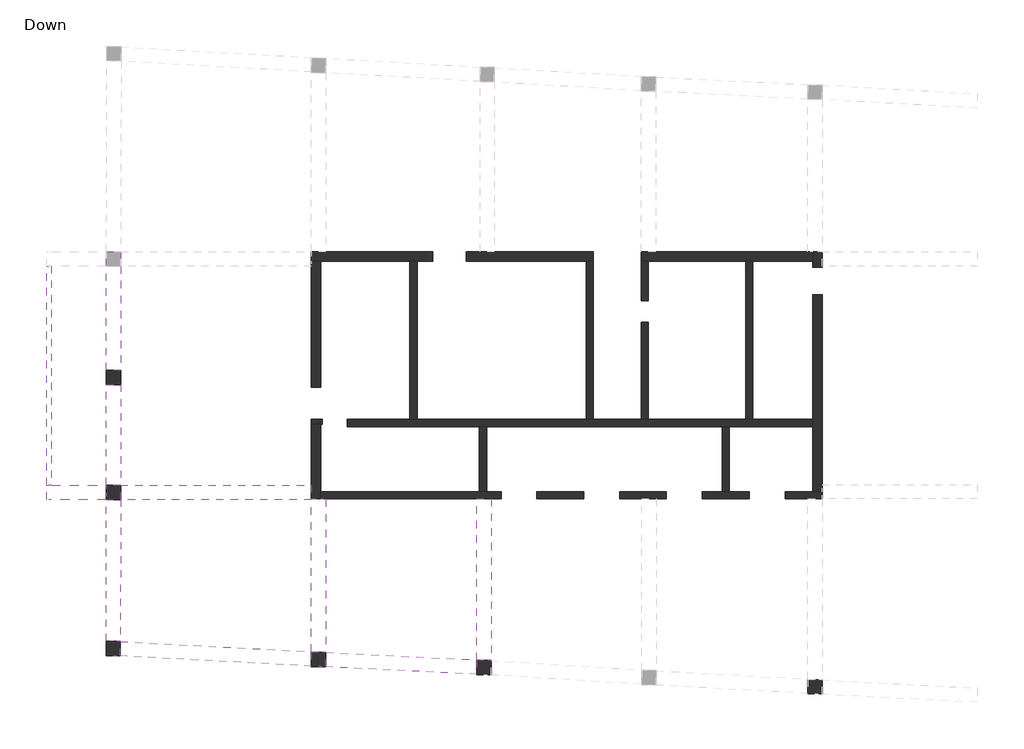
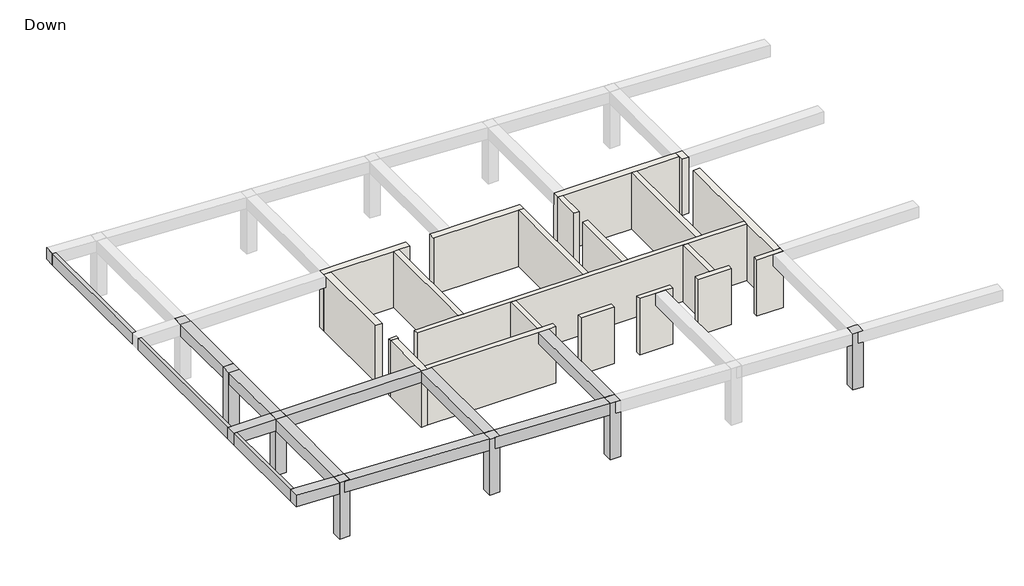
# One storey, part 1 of 2: 21 walls, 10 beams, 6 columns.
"""IFC4 building model written with IfcOpenShell, lengths in millimetres."""

from ifc_helpers import new_model, si_unit, origin, origin_with_axes, place, context, project, spatial, polyline, outline, extrude, faceted_brep, element, save

model = new_model("IFC4")

# Units and contexts
model_context = context("Model", 3, world=origin())
ifc_project = project(units=[si_unit("LENGTHUNIT", "METRE", prefix="MILLI")], contexts=[model_context])

# Site, building, storey
site = spatial("IfcSite", under=ifc_project)
building = spatial("IfcBuilding", under=site)
storey = spatial("IfcBuildingStorey", under=building, Name="Down", Elevation=0.0)

# Beams
placement = place(None, origin())
element("IfcBeam", 1, ObjectType="Concrete Rectengular Beam : 20/70", at=placement, inside=storey, context=model_context, shape_type="Brep", body=[
    faceted_brep([(-18610.0734048, 10852.5835779, 3500.0), (-18643.7818749, 10854.4803419, 3500.0), (-18643.7818749, 10253.5312104, 3500.0), (-18443.7818749, 10242.2772794, 2800.0), (-18443.7818749, 10242.2772794, 3250.0), (-18443.7818749, 10242.2772794, 3500.0), (-18443.7818749, 2137.8533878, 3500.0), (-18443.7818749, 2137.8533878, 3250.0), (-18443.7818749, 2137.8533878, 2800.0), (-18643.7818749, 10854.4803419, 2800.0), (-18610.0734048, 10852.5835779, 2800.0), (-18643.7818749, 10253.5312104, 2800.0), (-18643.7818749, 2137.8533878, 2800.0), (-18643.7818749, 2137.8533878, 3500.0)], [[[0, 1, 2]], [[3, 4, 5, 6, 7, 8]], [[9, 10, 11]], [[1, 9, 11, 12, 13, 2]], [[9, 1, 0, 10]], [[11, 2, 5, 4, 3]], [[2, 11, 10, 0]], [[5, 2, 13, 6]], [[11, 3, 8, 12]], [[8, 7, 6, 13, 12]]]),
    faceted_brep([(-18443.7818749, -13968.0424313, 2800.0), (-18443.7818749, -13968.0424313, 3250.0), (-18443.7818749, -13968.0424313, 3500.0), (-18643.7818749, -13957.4152549, 3500.0), (-18643.7818749, -13957.4152549, 2800.0), (-18443.7818749, -8198.714204, 3500.0), (-18443.7818749, -8198.714204, 3250.0), (-18443.7818749, -8198.714204, 2800.0), (-18643.7818749, -8198.714204, 2800.0), (-18643.7818749, -8198.714204, 3500.0)], [[[0, 1, 2, 3, 4]], [[5, 6, 7, 8, 9]], [[2, 1, 0, 7, 6, 5]], [[4, 3, 9, 8]], [[3, 2, 5, 9]], [[0, 4, 8, 7]]]),
    faceted_brep([(-18443.7818749, 1537.8533878, 3500.0), (-18443.7818749, 1537.8533878, 3250.0), (-18443.7818749, 1537.8533878, 2800.0), (-18643.7818749, 1537.8533878, 2800.0), (-18643.7818749, 1537.8533878, 3500.0), (-18443.7818749, -7598.714204, 3500.0), (-18443.7818749, -7598.714204, 3250.0), (-18443.7818749, -7598.714204, 2800.0), (-18643.7818749, -7598.714204, 2800.0), (-18643.7818749, -7598.714204, 3500.0)], [[[0, 1, 2, 3, 4]], [[2, 1, 0, 5, 6, 7]], [[4, 3, 8, 9]], [[0, 4, 9, 5]], [[3, 2, 7, 8]], [[7, 6, 5, 9, 8]]]),
])
element("IfcBeam", 2, ObjectType="Concrete Rectengular Beam : 60/70", at=placement, inside=storey, context=model_context, shape_type="Brep", body=[
    faceted_brep([(-702.7226745, -15484.7502418, 3500.0), (-702.7226745, -14899.1123715, 3500.0), (-395.3655019, -14899.1123715, 3500.0), (-702.7226745, -14884.028101, 3500.0), (-6997.0277588, -14575.1203917, 3500.0), (-6997.0277588, -15160.7582621, 3500.0), (-7304.3849313, -15160.7582621, 3500.0), (-395.3655019, -14899.1123715, 2800.0), (-702.7226745, -14884.028101, 2800.0), (-6997.0277588, -14575.1203917, 2800.0), (-6997.0277588, -14575.1203917, 3300.0), (-702.7226745, -14899.1123715, 2800.0), (-702.7226745, -15484.7502418, 2800.0), (-7304.3849313, -15160.7582621, 2800.0), (-6997.0277588, -15160.7582621, 2800.0)], [[[0, 1, 2, 3, 4, 5, 6]], [[2, 7, 8, 9, 10, 4, 3]], [[11, 12, 13, 14, 9, 8, 7]], [[12, 0, 6, 13]], [[11, 1, 0, 12]], [[1, 11, 7, 2]], [[14, 5, 4, 10, 9]], [[5, 14, 13, 6]]]),
])
element("IfcBeam", 3, ObjectType="Concrete Rectengular Beam : 60/70", at=placement, inside=storey, context=model_context, shape_type="Brep", body=[
    faceted_brep([(-16163.099747, -14690.0749183, 3500.0), (-16162.4709421, -14105.2863235, 3500.0), (-15854.6677574, -14105.6172946, 3500.0), (-16162.4537125, -14089.2628163, 3500.0), (-18443.7818749, -13968.0424313, 3500.0), (-18643.7818749, -13957.4152549, 3500.0), (-18643.7818749, -14558.2616844, 3500.0), (-15854.6677574, -14105.6172946, 2800.0), (-16162.4537125, -14089.2628163, 2800.0), (-18443.7818749, -13968.0424313, 2800.0), (-18643.7818749, -13957.4152549, 2800.0), (-16162.4709421, -14105.2863235, 2800.0), (-16163.099747, -14690.0749183, 2800.0), (-18643.7818749, -14558.2616844, 2800.0)], [[[0, 1, 2, 3, 4, 5, 6]], [[2, 7, 8, 9, 10, 5, 4, 3]], [[11, 12, 13, 10, 9, 8, 7]], [[12, 0, 6, 13]], [[11, 1, 0, 12]], [[1, 11, 7, 2]], [[6, 5, 10, 13]]]),
    faceted_brep([(-15563.1164499, -14705.9311375, 2800.0), (-15563.1164499, -14705.9311375, 3500.0), (-15562.4876449, -14121.1425427, 3500.0), (-15562.4876449, -14121.1425427, 3250.0), (-15562.4876449, -14121.1425427, 2800.0), (-15870.9196346, -14705.6001664, 2800.0), (-15870.9196346, -14705.6001664, 3500.0), (-7597.0277588, -14560.7582621, 2800.0), (-7597.0277588, -14560.7582621, 3500.0), (-7597.0277588, -15145.2407122, 3500.0), (-7597.0277588, -15145.2407122, 2800.0), (-7289.0629944, -14560.7582621, 2800.0), (-7289.0629944, -14560.7582621, 3500.0), (-7597.0277588, -14544.3942826, 3500.0), (-7597.0277588, -14544.3942826, 2800.0)], [[[0, 1, 2, 3, 4]], [[1, 0, 5, 6]], [[7, 8, 9, 10]], [[8, 7, 11, 12]], [[2, 1, 6, 9, 8, 12, 13]], [[12, 11, 14, 4, 3, 2, 13]], [[0, 4, 14, 11, 7, 10, 5]], [[6, 5, 10, 9]]]),
])
element("IfcBeam", 4, ObjectType="Concrete Rectengular Beam : 60/70", at=placement, inside=storey, context=model_context, shape_type="Brep", body=[
    faceted_brep([(-15556.1197891, -8199.036611, 3500.0), (-16156.1194422, -8198.3914501, 3500.0), (-16156.1197893, -8198.714204, 3500.0), (-16162.4537125, -14089.2628163, 3500.0), (-15854.6677574, -14105.6172946, 3500.0), (-15562.471289, -14105.9314844, 3500.0), (-15562.471289, -14105.9314844, 3250.0), (-15562.471289, -14105.9314844, 2800.0), (-15556.1197891, -8199.036611, 2800.0), (-15556.1197891, -8199.036611, 3250.0), (-16156.1194422, -8198.3914501, 2800.0), (-15854.6677574, -14105.6172946, 2800.0), (-16162.4537125, -14089.2628163, 2800.0), (-16156.1197893, -8198.714204, 2800.0), (-16162.4537125, -14089.2628163, 3250.0)], [[[0, 1, 2, 3, 4, 5]], [[0, 5, 6, 7, 8, 9]], [[10, 8, 7, 11, 12, 13]], [[1, 10, 13, 12, 14, 3, 2]], [[1, 0, 9, 8, 10]], [[4, 3, 14, 12, 11]], [[5, 4, 11, 7, 6]]]),
])
element("IfcBeam", 5, ObjectType="Concrete Rectengular Beam : 60/70", at=placement, inside=storey, context=model_context, shape_type="Brep", body=[
    faceted_brep([(-15550.9733173, -3412.8178686, 3500.0), (-16150.9729705, -3412.1727076, 3500.0), (-16155.4742813, -7598.391797, 3500.0), (-15555.4746282, -7599.0369579, 3500.0), (-15555.4742811, -7598.714204, 3500.0), (-15555.4746282, -7599.0369579, 2800.0), (-15550.9733173, -3412.8178686, 2800.0), (-15550.9733173, -3412.8178686, 3250.0), (-16150.9729705, -3412.1727076, 2800.0), (-16155.4742813, -7598.391797, 2800.0), (-16150.9729705, -3412.1727076, 3250.0), (-16155.4742813, -7598.391797, 3250.0)], [[[0, 1, 2, 3, 4]], [[5, 6, 7, 0, 4, 3]], [[8, 6, 5, 9]], [[2, 1, 10, 8, 9, 11]], [[1, 0, 7, 6, 8, 10]], [[3, 2, 11, 9, 5]]]),
])
element("IfcBeam", 6, ObjectType="Concrete Rectengular Beam : 60/70", at=placement, inside=storey, context=model_context, shape_type="Brep", body=[
    faceted_brep([(-16150.3278096, -2812.1730545, 3500.0), (-15550.3281564, -2812.8182154, 3500.0), (-15545.6500149, 1537.8533878, 3500.0), (-15545.0048536, 2137.8533878, 3500.0), (-16145.0052005, 2137.8533878, 3500.0), (-16145.6503618, 1537.8533878, 3500.0), (-15545.0048536, 2137.8533878, 2800.0), (-15550.3281564, -2812.8182154, 3250.0), (-15550.3281564, -2812.8182154, 2800.0), (-15545.6500149, 1537.8533878, 2800.0), (-16150.3278096, -2812.1730545, 2800.0), (-16145.6503618, 1537.8533878, 2800.0), (-16145.0052005, 2137.8533878, 2800.0), (-16150.3278096, -2812.1730545, 3250.0)], [[[0, 1, 2, 3, 4, 5]], [[6, 3, 2, 1, 7, 8, 9]], [[8, 10, 11, 12, 6, 9]], [[4, 12, 11, 10, 13, 0, 5]], [[1, 0, 13, 10, 8, 7]], [[4, 3, 6, 12]]]),
])
element("IfcBeam", 7, ObjectType="Concrete Rectengular Beam : 60/70", at=placement, inside=storey, context=model_context, shape_type="Brep", body=[
    faceted_brep([(-18643.7818749, -7598.714204, 3500.0), (-18643.7818749, -8198.714204, 3500.0), (-18443.7818749, -8198.714204, 3500.0), (-16156.1197893, -8198.714204, 3500.0), (-16156.1194422, -8198.3914501, 3500.0), (-16155.8039367, -7904.9712623, 3500.0), (-16155.474628, -7598.714204, 3500.0), (-18443.7818749, -7598.714204, 3500.0), (-16155.474628, -7598.714204, 3250.0), (-16155.474628, -7598.714204, 2800.0), (-18443.7818749, -7598.714204, 2800.0), (-18643.7818749, -7598.714204, 2800.0), (-18643.7818749, -8198.714204, 2800.0), (-16155.8039367, -7904.9712623, 2800.0), (-16156.1194422, -8198.3914501, 2800.0), (-16156.1197893, -8198.714204, 2800.0), (-18443.7818749, -8198.714204, 2800.0), (-16156.1197893, -8198.714204, 3250.0)], [[[0, 1, 2, 3, 4, 5, 6, 7]], [[6, 8, 9, 10, 11, 0, 7]], [[12, 11, 10, 9, 13, 14, 15, 16]], [[15, 17, 3, 2, 1, 12, 16]], [[3, 17, 15, 14, 13, 9, 8, 6, 5, 4]], [[1, 0, 11, 12]]]),
])
element("IfcBeam", 8, ObjectType="Concrete Rectengular Beam : 60/70", at=placement, inside=storey, context=model_context, shape_type="Brep", body=[
    faceted_brep([(-6997.0277588, -14560.7582621, 3500.0), (-6997.0277588, -8172.2965545, 3500.0), (-7199.5626242, -8172.2965545, 3500.0), (-7597.0277588, -8172.2965545, 3500.0), (-7597.0277588, -8198.714204, 3500.0), (-7597.0277588, -14544.3942826, 3500.0), (-7289.0629944, -14560.7582621, 3500.0), (-6997.0277588, -14560.7582621, 2800.0), (-6997.0277588, -8172.2965545, 2800.0), (-6997.0277588, -8172.2965545, 3300.0), (-7597.0277588, -8172.2965545, 2800.0), (-7289.0629944, -14560.7582621, 2800.0), (-7597.0277588, -14544.3942826, 2800.0), (-7597.0277588, -8198.714204, 2800.0), (-7597.0277588, -14544.3942826, 3250.0)], [[[0, 1, 2, 3, 4, 5, 6]], [[0, 7, 8, 9, 1]], [[10, 8, 7, 11, 12, 13]], [[12, 14, 5, 4, 3, 10, 13]], [[7, 0, 6, 11]], [[1, 9, 8, 10, 3, 2]], [[6, 5, 14, 12, 11]]]),
])
element("IfcBeam", 9, ObjectType="Concrete Rectengular Beam : 60/70", at=placement, inside=storey, context=model_context, shape_type="Brep", body=[
    faceted_brep([(-15555.4742811, -7598.714204, 3500.0), (-15555.4746282, -7599.0369579, 3500.0), (-15556.1194424, -8198.714204, 3500.0), (-7597.0277588, -8198.714204, 3500.0), (-7597.0277588, -8172.2965545, 3500.0), (-7599.5626242, -8172.2965545, 3500.0), (-7599.5626242, -7598.714204, 3500.0), (-15556.1194424, -8198.714204, 3250.0), (-15556.1194424, -8198.714204, 2800.0), (-7597.0277588, -8198.714204, 2800.0), (-7597.0277588, -8198.714204, 3250.0), (-15555.4746282, -7599.0369579, 2800.0), (-15555.4742811, -7598.714204, 2800.0), (-7599.5626242, -7598.714204, 2800.0), (-7599.5626242, -8172.2965545, 2800.0), (-7597.0277588, -8172.2965545, 2800.0), (-15555.4742811, -7598.714204, 3250.0), (-7599.5626242, -7598.714204, 3250.0)], [[[0, 1, 2, 3, 4, 5, 6]], [[2, 7, 8, 9, 10, 3]], [[8, 11, 12, 13, 14, 15, 9]], [[12, 16, 0, 6, 17, 13]], [[8, 7, 2, 1, 0, 16, 12, 11]], [[5, 14, 13, 17, 6]], [[14, 5, 4, 15]], [[4, 3, 10, 9, 15]]]),
])
element("IfcBeam", 10, ObjectType="Concrete Rectengular Beam : 60/70", at=placement, inside=storey, context=model_context, shape_type="Brep", body=[
    faceted_brep([(-702.7226745, -14884.028101, 3500.0), (-395.3655019, -14899.1123715, 3500.0), (-102.7226745, -14899.1123715, 3500.0), (-102.7226745, -8172.2965545, 3500.0), (-702.7226745, -8172.2965545, 3500.0), (-102.7226745, -14899.1123715, 2800.0), (-102.7226745, -8172.2965545, 2800.0), (-102.7226745, -8172.2965545, 3300.0), (-395.3655019, -14899.1123715, 2800.0), (-702.7226745, -14884.028101, 2800.0), (-702.7226745, -8172.2965545, 2800.0), (-702.7226745, -14884.028101, 3300.0), (-702.7226745, -8172.2965545, 3300.0)], [[[0, 1, 2, 3, 4]], [[2, 5, 6, 7, 3]], [[8, 9, 10, 6, 5]], [[9, 11, 0, 4, 12, 10]], [[0, 11, 9, 8, 1]], [[2, 1, 8, 5]], [[4, 3, 7, 6, 10, 12]]]),
])

# Columns
element("IfcColumn", 11, ObjectType="Concrete Rectengular Column : 60/60", at=placement, inside=storey, context=model_context, shape_type="SweptSolid", body=[
    extrude(outline(polyline([(-15550.3281564, -2812.8182154), (-15550.9733173, -3412.8178686), (-16150.9729705, -3412.1727076), (-16150.3278096, -2812.1730545), (-15550.3281564, -2812.8182154)])), origin_with_axes(), (0.0, 0.0, 1.0), 3500.0),
])
element("IfcColumn", 12, ObjectType="Concrete Rectengular Column : 60/60", at=placement, inside=storey, context=model_context, shape_type="Brep", body=[
    faceted_brep([(-15555.4746282, -7599.0369579, 0.0), (-15556.1197891, -8199.036611, 0.0), (-16156.1194422, -8198.3914501, 0.0), (-16155.4742813, -7598.391797, 0.0), (-15555.4746282, -7599.0369579, 3500.0), (-15556.1194424, -8198.714204, 3500.0), (-15556.1197891, -8199.036611, 3500.0), (-16156.1194422, -8198.3914501, 3500.0), (-16155.474628, -7598.714204, 3500.0), (-16155.4742813, -7598.391797, 3500.0)], [[[0, 1, 2, 3]], [[4, 5, 6, 1, 0]], [[6, 7, 2, 1]], [[7, 8, 9, 3, 2]], [[9, 4, 0, 3]], [[4, 9, 8, 7, 6, 5]]]),
])
element("IfcColumn", 13, ObjectType="Concrete Rectengular Column : 60/60", at=placement, inside=storey, context=model_context, shape_type="Brep", body=[
    faceted_brep([(-15562.471289, -14105.9314844, 0.0), (-15563.1164499, -14705.9311375, 0.0), (-16163.116103, -14705.2859766, 0.0), (-16162.4709421, -14105.2863235, 0.0), (-15562.471289, -14105.9314844, 3500.0), (-15562.4876449, -14121.1425427, 3500.0), (-15563.1164499, -14705.9311375, 3500.0), (-15562.471289, -14105.9314844, 2800.0), (-16163.116103, -14705.2859766, 3500.0), (-16162.4709421, -14105.2863235, 3500.0), (-15854.6677574, -14105.6172946, 3500.0)], [[[0, 1, 2, 3]], [[4, 5, 6, 1, 0, 7]], [[6, 8, 2, 1]], [[8, 9, 3, 2]], [[9, 10, 4, 7, 0, 3]], [[4, 10, 9, 8, 6, 5]]]),
])
element("IfcColumn", 14, ObjectType="Concrete Rectengular Column : 60/60", at=placement, inside=storey, context=model_context, shape_type="SweptSolid", body=[
    extrude(outline(polyline([(13698.0421838, -15707.1262254), (13698.0421838, -16307.1262254), (13098.0421838, -16307.1262254), (13098.0421838, -15707.1262254), (13698.0421838, -15707.1262254)])), origin_with_axes(), (0.0, 0.0, 1.0), 3500.0),
])
element("IfcColumn", 15, ObjectType="Concrete Rectengular Column : 60/60", at=placement, inside=storey, context=model_context, shape_type="Brep", body=[
    faceted_brep([(-102.7226745, -14899.1123715, 0.0), (-102.7226745, -15499.1123715, 0.0), (-702.7226745, -15499.1123715, 0.0), (-702.7226745, -14899.1123715, 0.0), (-102.7226745, -14899.1123715, 3500.0), (-102.7226745, -14916.8878336, 3500.0), (-102.7226745, -15499.1123715, 3500.0), (-702.7226745, -15499.1123715, 3500.0), (-702.7226745, -14899.1123715, 3500.0)], [[[0, 1, 2, 3]], [[4, 5, 6, 1, 0]], [[6, 7, 2, 1]], [[7, 8, 3, 2]], [[8, 4, 0, 3]], [[4, 8, 7, 6, 5]]]),
])
element("IfcColumn", 16, ObjectType="Concrete Rectengular Column : 60/60", at=placement, inside=storey, context=model_context, shape_type="Brep", body=[
    faceted_brep([(-6997.0277588, -14560.7582621, 0.0), (-6997.0277588, -15160.7582621, 0.0), (-7597.0277588, -15160.7582621, 0.0), (-7597.0277588, -14560.7582621, 0.0), (-6997.0277588, -14560.7582621, 3500.0), (-6997.0277588, -14575.1203917, 3500.0), (-6997.0277588, -15160.7582621, 3500.0), (-7597.0277588, -15160.7582621, 3500.0), (-7597.0277588, -14560.7582621, 3500.0)], [[[0, 1, 2, 3]], [[4, 5, 6, 1, 0]], [[6, 7, 2, 1]], [[7, 8, 3, 2]], [[8, 4, 0, 3]], [[4, 8, 7, 6, 5]]]),
])

# Walls
element("IfcWall", 17, ObjectType="20", at=placement, inside=storey, context=model_context, shape_type="Brep", body=[
    faceted_brep([(-7599.5626242, -5055.687558, 0.0), (-7199.5626242, -5055.687558, 0.0), (-7139.5626242, -5055.687558, 0.0), (-7139.5626242, -5055.687558, 3250.0), (-7139.5626242, -5055.687558, 3500.0), (-7199.5626242, -5055.687558, 3500.0), (-7599.5626242, -5055.687558, 3500.0), (-7599.5626242, -4855.687558, 0.0), (-7599.5626242, -4855.687558, 3250.0), (-7599.5626242, -4855.687558, 3500.0), (-7199.5626242, -4855.687558, 3500.0), (-7139.5626242, -4855.687558, 3500.0), (-7139.5626242, -4855.687558, 3250.0), (-7139.5626242, -4855.687558, 0.0)], [[[0, 1, 2, 3, 4, 5, 6]], [[7, 8, 9, 10, 11, 12, 13]], [[2, 1, 0, 7, 13]], [[4, 3, 2, 13, 12, 11]], [[6, 5, 4, 11, 10, 9]], [[0, 6, 9, 8, 7]]]),
])
element("IfcWall", 18, ObjectType="30", at=placement, inside=storey, context=model_context, shape_type="Brep", body=[
    faceted_brep([(-7199.5626242, -8172.2965545, 0.0), (309.3899821, -8172.2965545, 0.0), (309.3899821, -8172.2965545, 3300.0), (309.3899821, -8172.2965545, 3500.0), (-102.7226745, -8172.2965545, 3500.0), (-702.7226745, -8172.2965545, 3500.0), (-6997.0277588, -8172.2965545, 3500.0), (-7199.5626242, -8172.2965545, 3500.0), (-7199.5626242, -7872.2965545, 0.0), (-7199.5626242, -7872.2965545, 3500.0), (-591.6077111, -7872.2965545, 3500.0), (-291.6077111, -7872.2965545, 3500.0), (309.3899821, -7872.2965545, 3500.0), (309.3899821, -7872.2965545, 3300.0), (309.3899821, -7872.2965545, 0.0), (-291.6077111, -7872.2965545, 0.0), (-591.6077111, -7872.2965545, 0.0)], [[[0, 1, 2, 3, 4, 5, 6, 7]], [[8, 9, 10, 11, 12, 13, 14, 15, 16]], [[1, 0, 8, 16, 15, 14]], [[3, 2, 1, 14, 13, 12]], [[7, 6, 5, 4, 3, 12, 11, 10, 9]], [[0, 7, 9, 8]]]),
])
element("IfcWall", 19, ObjectType="30", at=placement, inside=storey, context=model_context, shape_type="Brep", body=[
    faceted_brep([(1808.0058991, -8172.2965545, 0.0), (3757.0255069, -8172.2965545, 0.0), (3757.0255069, -8172.2965545, 3300.0), (3757.0255069, -8172.2965545, 3500.0), (1808.0058991, -8172.2965545, 3500.0), (1808.0058991, -8172.2965545, 3300.0), (1808.0058991, -7872.2965545, 0.0), (1808.0058991, -7872.2965545, 3300.0), (1808.0058991, -7872.2965545, 3500.0), (3757.0255069, -7872.2965545, 3500.0), (3757.0255069, -7872.2965545, 3300.0), (3757.0255069, -7872.2965545, 0.0)], [[[0, 1, 2, 3, 4, 5]], [[6, 7, 8, 9, 10, 11]], [[1, 0, 6, 11]], [[3, 2, 1, 11, 10, 9]], [[4, 3, 9, 8]], [[0, 5, 4, 8, 7, 6]]]),
])
element("IfcWall", 20, ObjectType="30", at=placement, inside=storey, context=model_context, shape_type="Brep", body=[
    faceted_brep([(5255.6414239, -8172.2965545, 0.0), (7204.6610317, -8172.2965545, 0.0), (7204.6610317, -8172.2965545, 3250.0), (7204.6610317, -8172.2965545, 3500.0), (6772.0250706, -8172.2965545, 3500.0), (6172.0250706, -8172.2965545, 3500.0), (5255.6414239, -8172.2965545, 3500.0), (5255.6414239, -8172.2965545, 3300.0), (5255.6414239, -7872.2965545, 0.0), (5255.6414239, -7872.2965545, 3300.0), (5255.6414239, -7872.2965545, 3500.0), (7204.6610317, -7872.2965545, 3500.0), (7204.6610317, -7872.2965545, 3250.0), (7204.6610317, -7872.2965545, 0.0)], [[[0, 1, 2, 3, 4, 5, 6, 7]], [[8, 9, 10, 11, 12, 13]], [[1, 0, 8, 13]], [[3, 2, 1, 13, 12, 11]], [[6, 5, 4, 3, 11, 10]], [[0, 7, 6, 10, 9, 8]]]),
])
element("IfcWall", 21, ObjectType="30", at=placement, inside=storey, context=model_context, shape_type="Brep", body=[
    faceted_brep([(8703.2769487, -8172.2965545, 0.0), (10652.2965565, -8172.2965545, 0.0), (10652.2965565, -8172.2965545, 3250.0), (10652.2965565, -8172.2965545, 3500.0), (8703.2769487, -8172.2965545, 3500.0), (8703.2769487, -8172.2965545, 3250.0), (8703.2769487, -7872.2965545, 0.0), (8703.2769487, -7872.2965545, 3250.0), (8703.2769487, -7872.2965545, 3500.0), (9530.3819083, -7872.2965545, 3500.0), (9830.3819083, -7872.2965545, 3500.0), (10652.2965565, -7872.2965545, 3500.0), (10652.2965565, -7872.2965545, 3250.0), (10652.2965565, -7872.2965545, 0.0), (9830.3819083, -7872.2965545, 0.0), (9530.3819083, -7872.2965545, 0.0)], [[[0, 1, 2, 3, 4, 5]], [[6, 7, 8, 9, 10, 11, 12, 13, 14, 15]], [[1, 0, 6, 15, 14, 13]], [[3, 2, 1, 13, 12, 11]], [[4, 3, 11, 10, 9, 8]], [[0, 5, 4, 8, 7, 6]]]),
])
element("IfcWall", 22, ObjectType="30", at=placement, inside=storey, context=model_context, shape_type="Brep", body=[
    faceted_brep([(12150.9124735, -8172.2965545, 0.0), (13705.5837537, -8172.2965545, 0.0), (13705.5837537, -8172.2965545, 2800.0), (13705.5837537, -8172.2965545, 3500.0), (13105.5837537, -8172.2965545, 3500.0), (12150.9124735, -8172.2965545, 3500.0), (12150.9124735, -8172.2965545, 3250.0), (12150.9124735, -7872.2965545, 0.0), (12150.9124735, -7872.2965545, 3250.0), (12150.9124735, -7872.2965545, 3500.0), (13305.5837537, -7872.2965545, 3500.0), (13705.5837537, -7872.2965545, 3500.0), (13705.5837537, -7872.2965545, 0.0), (13305.5837537, -7872.2965545, 0.0)], [[[0, 1, 2, 3, 4, 5, 6]], [[7, 8, 9, 10, 11, 12, 13]], [[1, 0, 7, 13, 12]], [[5, 4, 3, 11, 10, 9]], [[0, 6, 5, 9, 8, 7]], [[3, 2, 1, 12, 11]]]),
])
element("IfcWall", 23, ObjectType="30", at=placement, inside=storey, context=model_context, shape_type="Brep", body=[
    faceted_brep([(-291.6077111, -7872.2965545, 0.0), (-291.6077111, -5155.687558, 0.0), (-291.6077111, -5155.687558, 3250.0), (-291.6077111, -5155.687558, 3500.0), (-291.6077111, -7872.2965545, 3500.0), (-291.6077111, -7872.2965545, 3250.0), (-591.6077111, -7872.2965545, 0.0), (-591.6077111, -7872.2965545, 3500.0), (-591.6077111, -5155.687558, 3500.0), (-591.6077111, -5155.687558, 0.0)], [[[0, 1, 2, 3, 4, 5]], [[6, 7, 8, 9]], [[1, 0, 6, 9]], [[4, 3, 8, 7]], [[3, 2, 1, 9, 8]], [[0, 5, 4, 7, 6]]]),
])
element("IfcWall", 24, ObjectType="30", at=placement, inside=storey, context=model_context, shape_type="Brep", body=[
    faceted_brep([(9830.3819083, -7872.2965545, 0.0), (9830.3819083, -5155.687558, 0.0), (9830.3819083, -5155.687558, 3250.0), (9830.3819083, -5155.687558, 3500.0), (9830.3819083, -7872.2965545, 3500.0), (9830.3819083, -7872.2965545, 3250.0), (9530.3819083, -7872.2965545, 0.0), (9530.3819083, -7872.2965545, 3250.0), (9530.3819083, -7872.2965545, 3500.0), (9530.3819083, -5155.687558, 3500.0), (9530.3819083, -5155.687558, 3250.0), (9530.3819083, -5155.687558, 0.0)], [[[0, 1, 2, 3, 4, 5]], [[6, 7, 8, 9, 10, 11]], [[1, 0, 6, 11]], [[4, 3, 9, 8]], [[3, 2, 1, 11, 10, 9]], [[0, 5, 4, 8, 7, 6]]]),
])
element("IfcWall", 25, ObjectType="30", at=placement, inside=storey, context=model_context, shape_type="Brep", body=[
    faceted_brep([(-3190.3793374, -4855.687558, 0.0), (-3190.3793374, 1737.8533878, 0.0), (-3190.3793374, 1737.8533878, 3250.0), (-3190.3793374, 1737.8533878, 3500.0), (-3190.3793374, -4855.687558, 3500.0), (-3190.3793374, -4855.687558, 3250.0), (-3490.3793374, -4855.687558, 0.0), (-3490.3793374, -4855.687558, 3250.0), (-3490.3793374, -4855.687558, 3500.0), (-3490.3793374, 1737.8533878, 3500.0), (-3490.3793374, 1737.8533878, 3250.0), (-3490.3793374, 1737.8533878, 0.0)], [[[0, 1, 2, 3, 4, 5]], [[6, 7, 8, 9, 10, 11]], [[1, 0, 6, 11]], [[4, 3, 9, 8]], [[0, 5, 4, 8, 7, 6]], [[3, 2, 1, 11, 10, 9]]]),
])
element("IfcWall", 26, ObjectType="30", at=placement, inside=storey, context=model_context, shape_type="Brep", body=[
    faceted_brep([(4155.2954031, -4855.687558, 0.0), (4155.2954031, 1737.8533878, 0.0), (4155.2954031, 1737.8533878, 3250.0), (4155.2954031, 1737.8533878, 3500.0), (4155.2954031, -4855.687558, 3500.0), (4155.2954031, -4855.687558, 3250.0), (3855.2954031, -4855.687558, 0.0), (3855.2954031, -4855.687558, 3250.0), (3855.2954031, -4855.687558, 3500.0), (3855.2954031, 1737.8533878, 3500.0), (3855.2954031, 1737.8533878, 3250.0), (3855.2954031, 1737.8533878, 0.0)], [[[0, 1, 2, 3, 4, 5]], [[6, 7, 8, 9, 10, 11]], [[1, 0, 6, 11]], [[4, 3, 9, 8]], [[0, 5, 4, 8, 7, 6]], [[3, 2, 1, 11, 10, 9]]]),
])
element("IfcWall", 27, ObjectType="30", at=placement, inside=storey, context=model_context, shape_type="Brep", body=[
    faceted_brep([(6456.4488056, 90.5638838, 0.0), (6456.4488056, 1737.8533878, 0.0), (6456.4488056, 1737.8533878, 3250.0), (6456.4488056, 1737.8533878, 3500.0), (6456.4488056, 90.5638838, 3500.0), (6456.4488056, 90.5638838, 3250.0), (6156.4488056, 90.5638838, 0.0), (6156.4488056, 90.5638838, 3250.0), (6156.4488056, 90.5638838, 3500.0), (6156.4488056, 1737.8533878, 3500.0), (6156.4488056, 1737.8533878, 0.0)], [[[0, 1, 2, 3, 4, 5]], [[6, 7, 8, 9, 10]], [[1, 0, 6, 10]], [[4, 3, 9, 8]], [[0, 5, 4, 8, 7, 6]], [[3, 2, 1, 10, 9]]]),
])
element("IfcWall", 28, ObjectType="30", at=placement, inside=storey, context=model_context, shape_type="Brep", body=[
    faceted_brep([(6156.4488056, -810.243498, 0.0), (6156.4488056, -4855.687558, 0.0), (6156.4488056, -4855.687558, 3250.0), (6156.4488056, -4855.687558, 3500.0), (6156.4488056, -810.243498, 3500.0), (6156.4488056, -810.243498, 3250.0), (6456.4488056, -810.243498, 0.0), (6456.4488056, -810.243498, 3250.0), (6456.4488056, -810.243498, 3500.0), (6456.4488056, -4855.687558, 3500.0), (6456.4488056, -4855.687558, 3250.0), (6456.4488056, -4855.687558, 0.0)], [[[0, 1, 2, 3, 4, 5]], [[6, 7, 8, 9, 10, 11]], [[1, 0, 6, 11]], [[4, 3, 9, 8]], [[0, 5, 4, 8, 7, 6]], [[3, 2, 1, 11, 10, 9]]]),
])
element("IfcWall", 29, ObjectType="30", at=placement, inside=storey, context=model_context, shape_type="Brep", body=[
    faceted_brep([(10507.8905588, 1737.8533878, 0.0), (10507.8905588, -4855.687558, 0.0), (10507.8905588, -4855.687558, 3250.0), (10507.8905588, -4855.687558, 3500.0), (10507.8905588, 1737.8533878, 3500.0), (10507.8905588, 1737.8533878, 3250.0), (10807.8905588, 1737.8533878, 0.0), (10807.8905588, 1737.8533878, 3500.0), (10807.8905588, -4855.687558, 3500.0), (10807.8905588, -4855.687558, 0.0)], [[[0, 1, 2, 3, 4, 5]], [[6, 7, 8, 9]], [[1, 0, 6, 9]], [[4, 3, 8, 7]], [[3, 2, 1, 9, 8]], [[0, 5, 4, 7, 6]]]),
])
element("IfcWall", 30, ObjectType="30", at=placement, inside=storey, context=model_context, shape_type="Brep", body=[
    faceted_brep([(13305.5837537, -4855.687558, 0.0), (10807.8905588, -4855.687558, 0.0), (10507.8905588, -4855.687558, 0.0), (6456.4488056, -4855.687558, 0.0), (6156.4488056, -4855.687558, 0.0), (4155.2954031, -4855.687558, 0.0), (3855.2954031, -4855.687558, 0.0), (-3190.3793374, -4855.687558, 0.0), (-3490.3793374, -4855.687558, 0.0), (-6094.5315865, -4855.687558, 0.0), (-6094.5315865, -4855.687558, 3250.0), (-6094.5315865, -4855.687558, 3500.0), (-3490.3793374, -4855.687558, 3500.0), (-3190.3793374, -4855.687558, 3500.0), (3855.2954031, -4855.687558, 3500.0), (4155.2954031, -4855.687558, 3500.0), (6156.4488056, -4855.687558, 3500.0), (6456.4488056, -4855.687558, 3500.0), (10507.8905588, -4855.687558, 3500.0), (10807.8905588, -4855.687558, 3500.0), (13305.5837537, -4855.687558, 3500.0), (13305.5837537, -5155.687558, 0.0), (13305.5837537, -5155.687558, 3250.0), (13305.5837537, -5155.687558, 3500.0), (9830.3819083, -5155.687558, 3500.0), (9530.3819083, -5155.687558, 3500.0), (-291.6077111, -5155.687558, 3500.0), (-591.6077111, -5155.687558, 3500.0), (-6094.5315865, -5155.687558, 3500.0), (-6094.5315865, -5155.687558, 3250.0), (-6094.5315865, -5155.687558, 0.0), (-591.6077111, -5155.687558, 0.0), (-291.6077111, -5155.687558, 0.0), (9530.3819083, -5155.687558, 0.0), (9830.3819083, -5155.687558, 0.0)], [[[0, 1, 2, 3, 4, 5, 6, 7, 8, 9, 10, 11, 12, 13, 14, 15, 16, 17, 18, 19, 20]], [[21, 22, 23, 24, 25, 26, 27, 28, 29, 30, 31, 32, 33, 34]], [[9, 8, 7, 6, 5, 4, 3, 2, 1, 0, 21, 34, 33, 32, 31, 30]], [[11, 10, 9, 30, 29, 28]], [[20, 19, 18, 17, 16, 15, 14, 13, 12, 11, 28, 27, 26, 25, 24, 23]], [[0, 20, 23, 22, 21]]]),
])
element("IfcWall", 31, ObjectType="40", at=placement, inside=storey, context=model_context, shape_type="Brep", body=[
    faceted_brep([(-7199.5626242, -8172.2965545, 0.0), (-7199.5626242, -7872.2965545, 0.0), (-7199.5626242, -5055.687558, 0.0), (-7199.5626242, -5055.687558, 3250.0), (-7199.5626242, -5055.687558, 3500.0), (-7199.5626242, -5155.687558, 3500.0), (-7199.5626242, -7872.2965545, 3500.0), (-7199.5626242, -8172.2965545, 3500.0), (-7599.5626242, -8172.2965545, 0.0), (-7599.5626242, -8172.2965545, 3500.0), (-7599.5626242, -7598.714204, 3500.0), (-7599.5626242, -5055.687558, 3500.0), (-7599.5626242, -5055.687558, 0.0), (-7597.0277588, -8172.2965545, 3500.0)], [[[0, 1, 2, 3, 4, 5, 6, 7]], [[8, 9, 10, 11, 12]], [[2, 1, 0, 8, 12]], [[7, 6, 5, 4, 11, 10, 9, 13]], [[4, 3, 2, 12, 11]], [[0, 7, 13, 9, 8]]]),
])
element("IfcWall", 32, ObjectType="40", at=placement, inside=storey, context=model_context, shape_type="Brep", body=[
    faceted_brep([(13705.5837537, -7872.2965545, 0.0), (13705.5837537, 336.2386242, 0.0), (13705.5837537, 336.2386242, 3250.0), (13705.5837537, 336.2386242, 3500.0), (13705.5837537, -7572.2965545, 3500.0), (13705.5837537, -7872.2965545, 3500.0), (13305.5837537, -7872.2965545, 0.0), (13305.5837537, -7872.2965545, 3250.0), (13305.5837537, -7872.2965545, 3500.0), (13305.5837537, -5155.687558, 3500.0), (13305.5837537, -4855.687558, 3500.0), (13305.5837537, 336.2386242, 3500.0), (13305.5837537, 336.2386242, 3250.0), (13305.5837537, 336.2386242, 0.0), (13305.5837537, -4855.687558, 0.0), (13305.5837537, -5155.687558, 0.0)], [[[0, 1, 2, 3, 4, 5]], [[6, 7, 8, 9, 10, 11, 12, 13, 14, 15]], [[1, 0, 6, 15, 14, 13]], [[3, 2, 1, 13, 12, 11]], [[5, 4, 3, 11, 10, 9, 8]], [[0, 5, 8, 7, 6]]]),
])
element("IfcWall", 33, ObjectType="40", at=placement, inside=storey, context=model_context, shape_type="Brep", body=[
    faceted_brep([(13705.5837537, 1490.9099045, 0.0), (13705.5837537, 2137.8533878, 0.0), (13705.5837537, 2137.8533878, 2800.0), (13705.5837537, 2137.8533878, 3500.0), (13705.5837537, 1537.8533878, 3500.0), (13705.5837537, 1490.9099045, 3500.0), (13705.5837537, 1490.9099045, 3250.0), (13305.5837537, 1490.9099045, 0.0), (13305.5837537, 1490.9099045, 3250.0), (13305.5837537, 1490.9099045, 3500.0), (13305.5837537, 1737.8533878, 3500.0), (13305.5837537, 2137.8533878, 3500.0), (13305.5837537, 2137.8533878, 0.0), (13305.5837537, 1737.8533878, 0.0)], [[[0, 1, 2, 3, 4, 5, 6]], [[7, 8, 9, 10, 11, 12, 13]], [[1, 0, 7, 13, 12]], [[5, 4, 3, 11, 10, 9]], [[0, 6, 5, 9, 8, 7]], [[3, 2, 1, 12, 11]]]),
])
element("IfcWall", 34, ObjectType="40", at=placement, inside=storey, context=model_context, shape_type="Brep", body=[
    faceted_brep([(13305.5837537, 2137.8533878, 0.0), (6156.4488056, 2137.8533878, 0.0), (6156.4488056, 2137.8533878, 3250.0), (6156.4488056, 2137.8533878, 3500.0), (6756.4488056, 2137.8533878, 3500.0), (13105.5837537, 2137.8533878, 3500.0), (13305.5837537, 2137.8533878, 3500.0), (13305.5837537, 1737.8533878, 0.0), (13305.5837537, 1737.8533878, 3500.0), (10807.8905588, 1737.8533878, 3500.0), (10507.8905588, 1737.8533878, 3500.0), (6456.4488056, 1737.8533878, 3500.0), (6156.4488056, 1737.8533878, 3500.0), (6156.4488056, 1737.8533878, 0.0), (6456.4488056, 1737.8533878, 0.0), (10507.8905588, 1737.8533878, 0.0), (10807.8905588, 1737.8533878, 0.0)], [[[0, 1, 2, 3, 4, 5, 6]], [[7, 8, 9, 10, 11, 12, 13, 14, 15, 16]], [[1, 0, 7, 16, 15, 14, 13]], [[6, 5, 4, 3, 12, 11, 10, 9, 8]], [[0, 6, 8, 7]], [[3, 2, 1, 13, 12]]]),
])
element("IfcWall", 35, ObjectType="40", at=placement, inside=storey, context=model_context, shape_type="Brep", body=[
    faceted_brep([(4158.2942497, 2137.8533878, 0.0), (-1148.2801448, 2137.8533878, 0.0), (-1148.2801448, 2137.8533878, 3250.0), (-1148.2801448, 2137.8533878, 3500.0), (-566.8499256, 2137.8533878, 3500.0), (33.1500744, 2137.8533878, 3500.0), (4158.2942497, 2137.8533878, 3500.0), (4158.2942497, 2137.8533878, 3250.0), (4158.2942497, 1737.8533878, 0.0), (4158.2942497, 1737.8533878, 3250.0), (4158.2942497, 1737.8533878, 3500.0), (4155.2954031, 1737.8533878, 3500.0), (3855.2954031, 1737.8533878, 3500.0), (-1148.2801448, 1737.8533878, 3500.0), (-1148.2801448, 1737.8533878, 3250.0), (-1148.2801448, 1737.8533878, 0.0), (3855.2954031, 1737.8533878, 0.0), (4155.2954031, 1737.8533878, 0.0), (-1148.2801448, 1752.8533878, 3500.0)], [[[0, 1, 2, 3, 4, 5, 6, 7]], [[8, 9, 10, 11, 12, 13, 14, 15, 16, 17]], [[1, 0, 8, 17, 16, 15]], [[3, 2, 1, 15, 14, 13, 18]], [[6, 5, 4, 3, 18, 13, 12, 11, 10]], [[0, 7, 6, 10, 9, 8]]]),
])
element("IfcWall", 36, ObjectType="40", at=placement, inside=storey, context=model_context, shape_type="Brep", body=[
    faceted_brep([(-2548.6261655, 2137.8533878, 0.0), (-7599.5626242, 2137.8533878, 0.0), (-7599.5626242, 2137.8533878, 2800.0), (-7599.5626242, 2137.8533878, 3500.0), (-6999.5626242, 2137.8533878, 3500.0), (-2548.6261655, 2137.8533878, 3500.0), (-2548.6261655, 2137.8533878, 3250.0), (-2548.6261655, 1737.8533878, 0.0), (-2548.6261655, 1737.8533878, 3250.0), (-2548.6261655, 1737.8533878, 3500.0), (-3190.3793374, 1737.8533878, 3500.0), (-3490.3793374, 1737.8533878, 3500.0), (-7199.5626242, 1737.8533878, 3500.0), (-7599.5626242, 1737.8533878, 3500.0), (-7599.5626242, 1737.8533878, 0.0), (-7199.5626242, 1737.8533878, 0.0), (-3490.3793374, 1737.8533878, 0.0), (-3190.3793374, 1737.8533878, 0.0), (-2548.6261655, 1752.8533878, 3500.0)], [[[0, 1, 2, 3, 4, 5, 6]], [[7, 8, 9, 10, 11, 12, 13, 14, 15, 16, 17]], [[1, 0, 7, 17, 16, 15, 14]], [[5, 4, 3, 13, 12, 11, 10, 9, 18]], [[0, 6, 5, 18, 9, 8, 7]], [[3, 2, 1, 14, 13]]]),
])
element("IfcWall", 37, ObjectType="40", at=placement, inside=storey, context=model_context, shape_type="Brep", body=[
    faceted_brep([(-7599.5626242, 1737.8533878, 0.0), (-7599.5626242, -3512.6656433, 0.0), (-7599.5626242, -3512.6656433, 3250.0), (-7599.5626242, -3512.6656433, 3500.0), (-7599.5626242, 1537.8533878, 3500.0), (-7599.5626242, 1737.8533878, 3500.0), (-7199.5626242, 1737.8533878, 0.0), (-7199.5626242, 1737.8533878, 3250.0), (-7199.5626242, 1737.8533878, 3500.0), (-7199.5626242, -3512.6656433, 3500.0), (-7199.5626242, -3512.6656433, 3250.0), (-7199.5626242, -3512.6656433, 0.0)], [[[0, 1, 2, 3, 4, 5]], [[6, 7, 8, 9, 10, 11]], [[1, 0, 6, 11]], [[3, 2, 1, 11, 10, 9]], [[5, 4, 3, 9, 8]], [[0, 5, 8, 7, 6]]]),
])

save(model, "model.ifc")

# Revit data of these elements
# Project information
#   Project Issue Date = "Issue Date"
#   Project Status = "Project Status"
#   Client Name = "לקוח"
#   Project Address = "Enter address here"
#   Project Name = "Project 046"
#   Project Number = "מספר פרויקט"
# Type "Concrete Rectengular Beam : 20/70"
#   Length [instance default] = 152.4 cm
#   b = 20 cm
#   h = 70 cm
#   Structural Material [instance default] = Concrete
#   Assembly Code = ""
# Type "Concrete Rectengular Beam : 60/70"
#   Length [instance default] = 152.4 cm
#   b = 60 cm
#   h = 70 cm
#   Structural Material [instance default] = Concrete
#   Assembly Code = ""
# Type "Concrete Rectengular Column : 60/60"
#   b = 60 cm
#   h = 60 cm
#   Structural Material [instance default] = Concrete
# Type "20"
#   Layers, outside or top first: 20 cm "Concrete" (function 1)
# Type "30"
#   Layers, outside or top first: 30 cm "Concrete" (function 1)
# Type "40"
#   Layers, outside or top first: 40 cm "Concrete" (function 1)
# Element 1 (IfcBeam, "Concrete Rectengular Beam : 20/70")
#   Comments = ""
#   Mark = "B1"
#   SOFiSTiK_AMG_Comments = ""
#   SOFiSTiK_AMG_Scheduled = yes
#   SOFiSTiK_AMG_Adjusted = yes
#   Structural Material = Concrete
#   Phase Created = New Construction
#   Materials on its faces: "Concrete"
# Element 2 (IfcBeam, "Concrete Rectengular Beam : 60/70")
#   Comments = ""
#   Mark = "B16"
#   SOFiSTiK_AMG_Comments = ""
#   SOFiSTiK_AMG_Scheduled = yes
#   SOFiSTiK_AMG_Adjusted = yes
#   Structural Material = Concrete
#   Phase Created = New Construction
#   Materials on its faces: "Concrete"
# Element 3 (IfcBeam, "Concrete Rectengular Beam : 60/70")
#   Comments = ""
#   Mark = "B17"
#   SOFiSTiK_AMG_Comments = ""
#   SOFiSTiK_AMG_Scheduled = yes
#   SOFiSTiK_AMG_Adjusted = yes
#   Structural Material = Concrete
#   Phase Created = New Construction
#   Materials on its faces: "Concrete"
# Element 4 (IfcBeam, "Concrete Rectengular Beam : 60/70")
#   Comments = ""
#   Mark = "B18"
#   SOFiSTiK_AMG_Comments = ""
#   SOFiSTiK_AMG_Scheduled = yes
#   SOFiSTiK_AMG_Adjusted = yes
#   Structural Material = Concrete
#   Phase Created = New Construction
#   Materials on its faces: "Concrete"
# Element 5 (IfcBeam, "Concrete Rectengular Beam : 60/70")
#   Comments = ""
#   Mark = "B19"
#   SOFiSTiK_AMG_Comments = ""
#   SOFiSTiK_AMG_Scheduled = yes
#   SOFiSTiK_AMG_Adjusted = yes
#   Structural Material = Concrete
#   Phase Created = New Construction
#   Materials on its faces: "Concrete"
# Element 6 (IfcBeam, "Concrete Rectengular Beam : 60/70")
#   Comments = ""
#   Mark = "B20"
#   SOFiSTiK_AMG_Comments = ""
#   SOFiSTiK_AMG_Scheduled = yes
#   SOFiSTiK_AMG_Adjusted = yes
#   Structural Material = Concrete
#   Phase Created = New Construction
#   Materials on its faces: "Concrete"
# Element 7 (IfcBeam, "Concrete Rectengular Beam : 60/70")
#   Comments = ""
#   Mark = "B26"
#   SOFiSTiK_AMG_Comments = ""
#   SOFiSTiK_AMG_Scheduled = yes
#   SOFiSTiK_AMG_Adjusted = yes
#   Structural Material = Concrete
#   Phase Created = New Construction
#   Materials on its faces: "Concrete"
# Element 8 (IfcBeam, "Concrete Rectengular Beam : 60/70")
#   Comments = ""
#   Mark = "B27"
#   SOFiSTiK_AMG_Comments = ""
#   SOFiSTiK_AMG_Scheduled = yes
#   SOFiSTiK_AMG_Adjusted = yes
#   Structural Material = Concrete
#   Phase Created = New Construction
#   Materials on its faces: "Concrete"
# Element 9 (IfcBeam, "Concrete Rectengular Beam : 60/70")
#   Comments = ""
#   Mark = "B28"
#   SOFiSTiK_AMG_Comments = ""
#   SOFiSTiK_AMG_Scheduled = yes
#   SOFiSTiK_AMG_Adjusted = yes
#   Structural Material = Concrete
#   Phase Created = New Construction
#   Materials on its faces: "Concrete"
# Element 10 (IfcBeam, "Concrete Rectengular Beam : 60/70")
#   Comments = ""
#   Mark = "B38"
#   SOFiSTiK_AMG_Comments = ""
#   SOFiSTiK_AMG_Scheduled = yes
#   SOFiSTiK_AMG_Adjusted = yes
#   Structural Material = Concrete
#   Phase Created = New Construction
#   Materials on its faces: "Concrete"
# Element 11 (IfcColumn, "Concrete Rectengular Column : 60/60")
#   Comments = ""
#   Mark = "C6"
#   SOFiSTiK_AMG_Comments = ""
#   SOFiSTiK_AMG_Scheduled = yes
#   SOFiSTiK_AMG_Adjusted = yes
#   Structural Material = Concrete
#   Phase Created = New Construction
#   Materials on its faces: "Concrete"
# Element 12 (IfcColumn, "Concrete Rectengular Column : 60/60")
#   Comments = ""
#   Mark = "C7"
#   SOFiSTiK_AMG_Comments = ""
#   SOFiSTiK_AMG_Scheduled = yes
#   SOFiSTiK_AMG_Adjusted = yes
#   Structural Material = Concrete
#   Phase Created = New Construction
#   Materials on its faces: "Concrete"
# Element 13 (IfcColumn, "Concrete Rectengular Column : 60/60")
#   Comments = ""
#   Mark = "C8"
#   SOFiSTiK_AMG_Comments = ""
#   SOFiSTiK_AMG_Scheduled = yes
#   SOFiSTiK_AMG_Adjusted = yes
#   Structural Material = Concrete
#   Phase Created = New Construction
#   Materials on its faces: "Concrete"
# Element 14 (IfcColumn, "Concrete Rectengular Column : 60/60")
#   Comments = ""
#   Mark = "C15"
#   SOFiSTiK_AMG_Comments = ""
#   SOFiSTiK_AMG_Scheduled = yes
#   SOFiSTiK_AMG_Adjusted = yes
#   Structural Material = Concrete
#   Phase Created = New Construction
#   Materials on its faces: "Concrete"
# Element 15 (IfcColumn, "Concrete Rectengular Column : 60/60")
#   Comments = ""
#   Mark = "C17"
#   SOFiSTiK_AMG_Comments = ""
#   SOFiSTiK_AMG_Scheduled = yes
#   SOFiSTiK_AMG_Adjusted = yes
#   Structural Material = Concrete
#   Phase Created = New Construction
#   Materials on its faces: "Concrete"
# Element 16 (IfcColumn, "Concrete Rectengular Column : 60/60")
#   Comments = ""
#   Mark = "C18"
#   SOFiSTiK_AMG_Comments = ""
#   SOFiSTiK_AMG_Scheduled = yes
#   SOFiSTiK_AMG_Adjusted = yes
#   Structural Material = Concrete
#   Phase Created = New Construction
#   Materials on its faces: "Concrete"
# Element 17 (IfcWall, "20")
#   Comments = ""
#   Mark = "W8"
#   SOFiSTiK_EdgeZones = "W8"
#   SOFiSTiK_AMG_Comments = ""
#   Top Offset = 0 cm
#   Base Offset = 0 cm
#   wall height = 350 cm
#   SOFiSTiK_AMG_Scheduled = yes
#   SOFiSTiK_AMG_Adjusted = yes
#   Phase Created = New Construction
#   Base Constraint = Down
#   Top Constraint = Typical Floor
#   Materials on its faces: "Concrete"
# Element 18 (IfcWall, "30")
#   Comments = ""
#   Mark = "W9"
#   SOFiSTiK_EdgeZones = "W9"
#   SOFiSTiK_AMG_Comments = ""
#   Top Offset = 0 cm
#   Base Offset = 0 cm
#   wall height = 350 cm
#   SOFiSTiK_AMG_Scheduled = yes
#   SOFiSTiK_AMG_Adjusted = yes
#   Phase Created = New Construction
#   Base Constraint = Down
#   Top Constraint = Typical Floor
#   Materials on its faces: "Concrete"
# Element 19 (IfcWall, "30")
#   Comments = ""
#   Mark = "W10"
#   SOFiSTiK_EdgeZones = "W10"
#   SOFiSTiK_AMG_Comments = ""
#   Top Offset = 0 cm
#   Base Offset = 0 cm
#   wall height = 350 cm
#   SOFiSTiK_AMG_Scheduled = yes
#   SOFiSTiK_AMG_Adjusted = yes
#   Phase Created = New Construction
#   Base Constraint = Down
#   Top Constraint = Typical Floor
#   Materials on its faces: "Concrete"
# Element 20 (IfcWall, "30")
#   Comments = ""
#   Mark = "W11"
#   SOFiSTiK_EdgeZones = "W11"
#   SOFiSTiK_AMG_Comments = ""
#   Top Offset = 0 cm
#   Base Offset = 0 cm
#   wall height = 350 cm
#   SOFiSTiK_AMG_Scheduled = yes
#   SOFiSTiK_AMG_Adjusted = yes
#   Phase Created = New Construction
#   Base Constraint = Down
#   Top Constraint = Typical Floor
#   Materials on its faces: "Concrete"
# Element 21 (IfcWall, "30")
#   Comments = ""
#   Mark = "W12"
#   SOFiSTiK_EdgeZones = "W12"
#   SOFiSTiK_AMG_Comments = ""
#   Top Offset = 0 cm
#   Base Offset = 0 cm
#   wall height = 350 cm
#   SOFiSTiK_AMG_Scheduled = yes
#   SOFiSTiK_AMG_Adjusted = yes
#   Phase Created = New Construction
#   Base Constraint = Down
#   Top Constraint = Typical Floor
#   Materials on its faces: "Concrete"
# Element 22 (IfcWall, "30")
#   Comments = ""
#   Mark = "W13"
#   SOFiSTiK_EdgeZones = "W13"
#   SOFiSTiK_AMG_Comments = ""
#   Top Offset = 0 cm
#   Base Offset = 0 cm
#   wall height = 350 cm
#   SOFiSTiK_AMG_Scheduled = yes
#   SOFiSTiK_AMG_Adjusted = yes
#   Phase Created = New Construction
#   Base Constraint = Down
#   Top Constraint = Typical Floor
#   Materials on its faces: "Concrete"
# Element 23 (IfcWall, "30")
#   Comments = ""
#   Mark = "W14"
#   SOFiSTiK_EdgeZones = "W14"
#   SOFiSTiK_AMG_Comments = ""
#   Top Offset = 0 cm
#   Base Offset = 0 cm
#   wall height = 350 cm
#   SOFiSTiK_AMG_Scheduled = yes
#   SOFiSTiK_AMG_Adjusted = yes
#   Phase Created = New Construction
#   Base Constraint = Down
#   Top Constraint = Typical Floor
#   Materials on its faces: "Concrete"
# Element 24 (IfcWall, "30")
#   Comments = ""
#   Mark = "W15"
#   SOFiSTiK_EdgeZones = "W15"
#   SOFiSTiK_AMG_Comments = ""
#   Top Offset = 0 cm
#   Base Offset = 0 cm
#   wall height = 350 cm
#   SOFiSTiK_AMG_Scheduled = yes
#   SOFiSTiK_AMG_Adjusted = yes
#   Phase Created = New Construction
#   Base Constraint = Down
#   Top Constraint = Typical Floor
#   Materials on its faces: "Concrete"
# Element 25 (IfcWall, "30")
#   Comments = ""
#   Mark = "W16"
#   SOFiSTiK_EdgeZones = "W16"
#   SOFiSTiK_AMG_Comments = ""
#   Top Offset = 0 cm
#   Base Offset = 0 cm
#   wall height = 350 cm
#   SOFiSTiK_AMG_Scheduled = yes
#   SOFiSTiK_AMG_Adjusted = yes
#   Phase Created = New Construction
#   Base Constraint = Down
#   Top Constraint = Typical Floor
#   Materials on its faces: "Concrete"
# Element 26 (IfcWall, "30")
#   Comments = ""
#   Mark = "W17"
#   SOFiSTiK_EdgeZones = "W17"
#   SOFiSTiK_AMG_Comments = ""
#   Top Offset = 0 cm
#   Base Offset = 0 cm
#   wall height = 350 cm
#   SOFiSTiK_AMG_Scheduled = yes
#   SOFiSTiK_AMG_Adjusted = yes
#   Phase Created = New Construction
#   Base Constraint = Down
#   Top Constraint = Typical Floor
#   Materials on its faces: "Concrete"
# Element 27 (IfcWall, "30")
#   Comments = ""
#   Mark = "W18"
#   SOFiSTiK_EdgeZones = "W18"
#   SOFiSTiK_AMG_Comments = ""
#   Top Offset = 0 cm
#   Base Offset = 0 cm
#   wall height = 350 cm
#   SOFiSTiK_AMG_Scheduled = yes
#   SOFiSTiK_AMG_Adjusted = yes
#   Phase Created = New Construction
#   Base Constraint = Down
#   Top Constraint = Typical Floor
#   Materials on its faces: "Concrete"
# Element 28 (IfcWall, "30")
#   Comments = ""
#   Mark = "W19"
#   SOFiSTiK_EdgeZones = "W19"
#   SOFiSTiK_AMG_Comments = ""
#   Top Offset = 0 cm
#   Base Offset = 0 cm
#   wall height = 350 cm
#   SOFiSTiK_AMG_Scheduled = yes
#   SOFiSTiK_AMG_Adjusted = yes
#   Phase Created = New Construction
#   Base Constraint = Down
#   Top Constraint = Typical Floor
#   Materials on its faces: "Concrete"
# Element 29 (IfcWall, "30")
#   Comments = ""
#   Mark = "W20"
#   SOFiSTiK_EdgeZones = "W20"
#   SOFiSTiK_AMG_Comments = ""
#   Top Offset = 0 cm
#   Base Offset = 0 cm
#   wall height = 350 cm
#   SOFiSTiK_AMG_Scheduled = yes
#   SOFiSTiK_AMG_Adjusted = yes
#   Phase Created = New Construction
#   Base Constraint = Down
#   Top Constraint = Typical Floor
#   Materials on its faces: "Concrete"
# Element 30 (IfcWall, "30")
#   Comments = ""
#   Mark = "W21"
#   SOFiSTiK_EdgeZones = "W21"
#   SOFiSTiK_AMG_Comments = ""
#   Top Offset = 0 cm
#   Base Offset = 0 cm
#   wall height = 350 cm
#   SOFiSTiK_AMG_Scheduled = yes
#   SOFiSTiK_AMG_Adjusted = yes
#   Phase Created = New Construction
#   Base Constraint = Down
#   Top Constraint = Typical Floor
#   Materials on its faces: "Concrete"
# Element 31 (IfcWall, "40")
#   Comments = ""
#   Mark = "W1"
#   SOFiSTiK_EdgeZones = "W1"
#   SOFiSTiK_AMG_Comments = ""
#   Top Offset = 0 cm
#   Base Offset = 0 cm
#   wall height = 350 cm
#   SOFiSTiK_AMG_Scheduled = yes
#   SOFiSTiK_AMG_Adjusted = yes
#   Phase Created = New Construction
#   Base Constraint = Down
#   Top Constraint = Typical Floor
#   Materials on its faces: "Concrete"
# Element 32 (IfcWall, "40")
#   Comments = ""
#   Mark = "W2"
#   SOFiSTiK_EdgeZones = "W2"
#   SOFiSTiK_AMG_Comments = ""
#   Top Offset = 0 cm
#   Base Offset = 0 cm
#   wall height = 350 cm
#   SOFiSTiK_AMG_Scheduled = yes
#   SOFiSTiK_AMG_Adjusted = yes
#   Phase Created = New Construction
#   Base Constraint = Down
#   Top Constraint = Typical Floor
#   Materials on its faces: "Concrete"
# Element 33 (IfcWall, "40")
#   Comments = ""
#   Mark = "W3"
#   SOFiSTiK_EdgeZones = "W3"
#   SOFiSTiK_AMG_Comments = ""
#   Top Offset = 0 cm
#   Base Offset = 0 cm
#   wall height = 350 cm
#   SOFiSTiK_AMG_Scheduled = yes
#   SOFiSTiK_AMG_Adjusted = yes
#   Phase Created = New Construction
#   Base Constraint = Down
#   Top Constraint = Typical Floor
#   Materials on its faces: "Concrete"
# Element 34 (IfcWall, "40")
#   Comments = ""
#   Mark = "W4"
#   SOFiSTiK_EdgeZones = "W4"
#   SOFiSTiK_AMG_Comments = ""
#   Top Offset = 0 cm
#   Base Offset = 0 cm
#   wall height = 350 cm
#   SOFiSTiK_AMG_Scheduled = yes
#   SOFiSTiK_AMG_Adjusted = yes
#   Phase Created = New Construction
#   Base Constraint = Down
#   Top Constraint = Typical Floor
#   Materials on its faces: "Concrete"
# Element 35 (IfcWall, "40")
#   Comments = ""
#   Mark = "W5"
#   SOFiSTiK_EdgeZones = "W5"
#   SOFiSTiK_AMG_Comments = ""
#   Top Offset = 0 cm
#   Base Offset = 0 cm
#   wall height = 350 cm
#   SOFiSTiK_AMG_Scheduled = yes
#   SOFiSTiK_AMG_Adjusted = yes
#   Phase Created = New Construction
#   Base Constraint = Down
#   Top Constraint = Typical Floor
#   Materials on its faces: "Concrete"
# Element 36 (IfcWall, "40")
#   Comments = ""
#   Mark = "W6"
#   SOFiSTiK_EdgeZones = "W6"
#   SOFiSTiK_AMG_Comments = ""
#   Top Offset = 0 cm
#   Base Offset = 0 cm
#   wall height = 350 cm
#   SOFiSTiK_AMG_Scheduled = yes
#   SOFiSTiK_AMG_Adjusted = yes
#   Phase Created = New Construction
#   Base Constraint = Down
#   Top Constraint = Typical Floor
#   Materials on its faces: "Concrete"
# Element 37 (IfcWall, "40")
#   Comments = ""
#   Mark = "W7"
#   SOFiSTiK_EdgeZones = "W7"
#   SOFiSTiK_AMG_Comments = ""
#   Top Offset = 0 cm
#   Base Offset = 0 cm
#   wall height = 350 cm
#   SOFiSTiK_AMG_Scheduled = yes
#   SOFiSTiK_AMG_Adjusted = yes
#   Phase Created = New Construction
#   Base Constraint = Down
#   Top Constraint = Typical Floor
#   Materials on its faces: "Concrete"
# Materials
#   "Concrete": class "Concrete", colour RGB 192 192 192, transparency 0, Keynote = "01000", Description = "Cast-in-place concrete", Cost = 0
